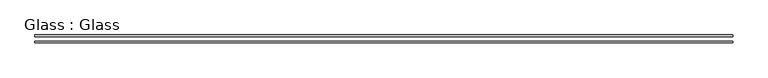
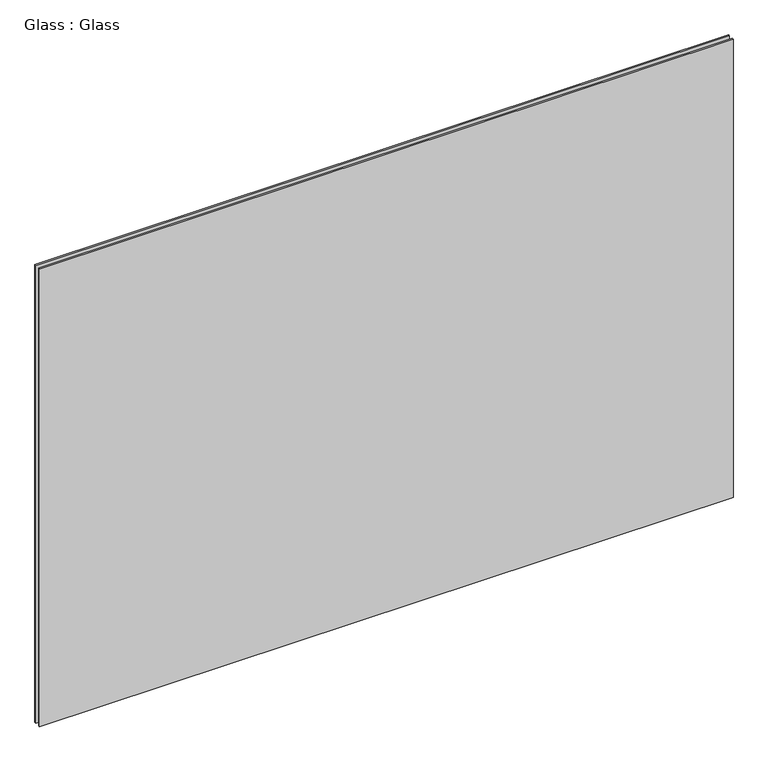
"""IFC4 building model written with IfcOpenShell, lengths in millimetres: proxy geometry, Glass : Glass."""

from ifc_helpers import new_model, si_unit, frame, origin, place, context, project, spatial, polyline, outline, extrude, source, transform, mapped, element, save


def glass_glass_7f8999f5(model_context):
    return source(origin(), model_context, "Body", "SweptSolid", [
        extrude(outline(polyline([(14383.0178845, -4394.1834255), (14383.0178845, -4398.9459255), (12383.0178845, -4398.9459255), (12383.0178845, -4394.1834255), (14383.0178845, -4394.1834255)])), frame((0.0, 0.0, 41130.5392812), z_axis=(0.0, 0.0, 1.0), x_axis=(1.0, 0.0, 0.0)), (0.0, 0.0, 1.0), 1396.8024401),
        extrude(outline(polyline([(14383.0178845, -4412.1834255), (14383.0178845, -4416.9459255), (12383.0178845, -4416.9459255), (12383.0178845, -4412.1834255), (14383.0178845, -4412.1834255)])), frame((0.0, 0.0, 41130.5392812), z_axis=(0.0, 0.0, 1.0), x_axis=(1.0, 0.0, 0.0)), (0.0, 0.0, 1.0), 1396.8024401),
    ])


if __name__ == "__main__":
    model = new_model("IFC4")
    model_context = context("Model", 3, world=origin())
    ifc_project = project(units=[si_unit("LENGTHUNIT", "METRE", prefix="MILLI")], contexts=[model_context])
    site = spatial("IfcSite", under=ifc_project)
    building = spatial("IfcBuilding", under=site)
    placement = place(None, origin())
    glass_glass_shape = glass_glass_7f8999f5(model_context)
    element("IfcBuildingElementProxy", 1, Name="Glass : Glass", ObjectType="Glass : Glass", at=placement, inside=building, context=model_context, shape_type="MappedRepresentation", body=[
        mapped(glass_glass_shape, transform((0.0, 0.0, 0.0), x_axis=(1.0, 0.0, 0.0), y_axis=(0.0, 1.0, 0.0), z_axis=(0.0, 0.0, 1.0))),
    ])
    save(model, "model.ifc")

# Revit data of these elements
# Type "Glass : Glass"
#   NameOverride = "Glass"
# Element 1 (IfcBuildingElementProxy, "Glass : Glass")
#   Materials on its faces: "1\"  INSULATED GLAZING"
# Materials
#   "1\"  INSULATED GLAZING": class "Unassigned", colour RGB 146 199 212, transparency 0, Cost = 0
